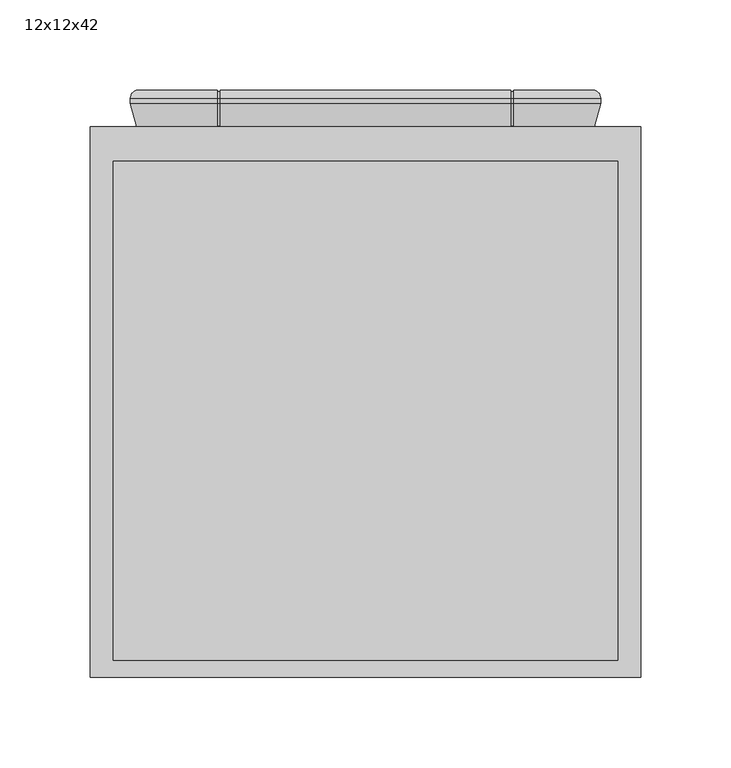
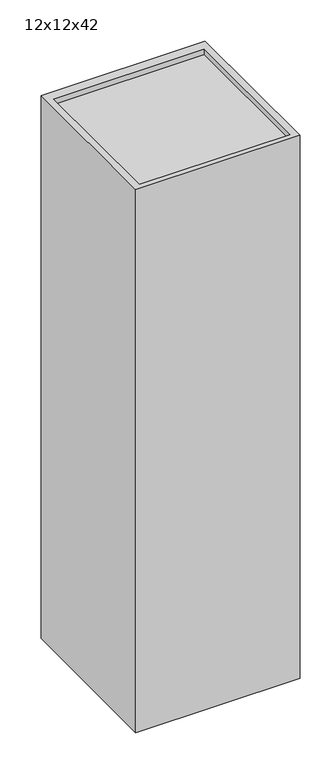
"""IFC4 building model written with IfcOpenShell, lengths in millimetres: furniture geometry, Cabinet-Wall-Merillat-Single_Door-Marlin : 12x12x42."""

from ifc_helpers import new_model, si_unit, frame, origin, place, context, project, spatial, polyline, circle_curve, ellipse_curve, outline, extrude, faceted_brep, source, transform, mapped, element, save
from ifc_brep_helpers import plane_surface, cylinder_surface, advanced_brep


def furniture_12x12x42_3f69c235(model_context):
    return source(origin(), model_context, "Body", "SolidModel", [
        advanced_brep(
        [(-100.4038372, 382.5621, 2108.2), (-97.3073447, 387.0325, 2105.1035075), (-97.3073447, 387.0325, 1095.2964925), (-100.4038372, 382.5621, 1092.2), (-100.4038372, 379.7935, 1092.2), (-100.4038372, 379.7935, 2108.2), (-96.8986372, 366.7125, 1095.7052), (-96.8986372, 366.7125, 2104.6948), (-52.2026744, 366.7125, 2059.9988372), (-52.2026744, 366.7125, 1140.4011628), (-51.8325427, 367.50625, 1140.7712945), (-49.7513837, 371.96931, 1142.8524535), (-49.7513837, 371.96931, 2057.5475465), (-51.8325427, 367.50625, 2059.6287055), (-51.1511532, 374.2094093, 1141.452684), (-51.1511532, 374.2094093, 2058.947316), (-65.4788372, 374.4595, 1127.125), (-65.4788372, 374.4595, 2073.275), (-65.4788372, 379.2855, 1127.125), (-65.4788372, 379.2855, 2073.275), (-51.1511532, 379.5355907, 1141.452684), (-51.1511532, 379.5355907, 2058.947316), (-49.7513837, 381.77569, 1142.8524535), (-49.7513837, 381.77569, 2057.5475465), (-51.8325427, 386.23875, 1140.7712945), (-52.199807, 387.0263508, 1140.4040302), (-52.2026744, 387.0325, 2059.9988372), (-51.8325427, 386.23875, 2059.6287055), (-52.199807, 387.0325, 1095.2964925), (-52.199807, 382.5621, 1092.2), (156.8496703, 387.0325, 1095.2964925), (159.9461628, 382.5621, 1092.2), (111.7819441, 382.5621, 1092.2), (111.7819441, 387.0325, 1095.2964925), (-50.612307, 382.5621, 1092.2), (-50.612307, 387.0325, 1095.2964925), (110.1944441, 387.0325, 1095.2964925), (110.1944441, 382.5621, 1092.2), (-52.199807, 379.7935, 1092.2), (159.9461628, 379.7935, 1092.2), (111.7819441, 379.7935, 1092.2), (-50.612307, 379.7935, 1092.2), (110.1944441, 379.7935, 1092.2), (-52.199807, 366.7125, 1095.7052), (156.4409628, 366.7125, 1095.7052), (111.7819441, 366.7125, 1095.7052), (-50.612307, 366.7125, 1095.7052), (110.1944441, 366.7125, 1095.7052), (109.2937093, 371.96931, 1142.8524535), (-50.612307, 367.50625, 1140.7712945), (-50.612307, 366.7125, 1140.4011628), (110.1944441, 366.7125, 1140.4011628), (110.1944441, 367.50625, 1140.7712945), (111.3748683, 367.50625, 1140.7712945), (110.6934787, 374.2094093, 1141.452684), (125.0211628, 374.4595, 1127.125), (125.0211628, 379.2855, 1127.125), (110.6934787, 379.5355907, 1141.452684), (109.2937093, 381.77569, 1142.8524535), (111.3748683, 386.23875, 1140.7712945), (110.1944441, 386.23875, 1140.7712945), (110.1944441, 387.0325, 1140.4011628), (-50.612307, 387.0325, 1140.4011628), (-50.612307, 386.23875, 1140.7712945), (156.8496703, 387.0325, 2105.1035075), (159.9461628, 382.5621, 2108.2), (159.9461628, 379.7935, 2108.2), (156.4409628, 366.7125, 2104.6948), (111.745, 366.7125, 1140.4011628), (111.745, 366.7125, 2059.9988372), (111.3748683, 367.50625, 2059.6287055), (109.2937093, 371.96931, 2057.5475465), (110.6934787, 374.2094093, 2058.947316), (125.0211628, 374.4595, 2073.275), (125.0211628, 379.2855, 2073.275), (110.6934787, 379.5355907, 2058.947316), (109.2937093, 381.77569, 2057.5475465), (111.3748683, 386.23875, 2059.6287055), (111.745, 387.0325, 2059.9988372), (111.745, 387.0325, 1140.4011628), (111.7819441, 387.0325, 2105.1035075), (111.7819441, 382.5621, 2108.2), (-52.199807, 382.5621, 2108.2), (-52.199807, 387.0325, 2105.1035075), (110.1944441, 382.5621, 2108.2), (110.1944441, 387.0325, 2105.1035075), (-50.612307, 387.0325, 2105.1035075), (-50.612307, 382.5621, 2108.2), (111.7819441, 379.7935, 2108.2), (-52.199807, 379.7935, 2108.2), (110.1944441, 379.7935, 2108.2), (-50.612307, 379.7935, 2108.2), (111.7819441, 366.7125, 2104.6948), (-52.199807, 366.7125, 2104.6948), (110.1944441, 366.7125, 2104.6948), (-50.612307, 366.7125, 2104.6948), (110.1944441, 366.7125, 2059.9988372), (-50.612307, 366.7125, 2059.9988372), (110.1944441, 367.50625, 2059.6287055), (-50.612307, 367.50625, 2059.6287055), (-50.612307, 386.23875, 2059.6287055), (-50.612307, 387.0325, 2059.9988372), (110.1944441, 387.0325, 2059.9988372), (110.1944441, 386.23875, 2059.6287055), (110.1944441, 367.50625, 2104.0857412), (110.1944441, 379.8980037, 2107.40625), (110.1944441, 382.5621, 2107.40625), (110.1944441, 386.23875, 2104.9526052), (111.7819441, 386.23875, 2059.6287055), (111.7819441, 386.23875, 2104.9526052), (111.7819441, 382.5621, 2107.40625), (111.7819441, 379.8980037, 2107.40625), (111.7819441, 367.50625, 2104.0857412), (111.7819441, 367.50625, 2059.6287055), (-52.199807, 367.50625, 2059.6287055), (-52.199807, 367.50625, 2104.0857412), (-52.199807, 379.8980037, 2107.40625), (-52.199807, 382.5621, 2107.40625), (-52.199807, 386.23875, 2104.9526052), (-52.199807, 386.23875, 2059.6287055), (-50.612307, 386.23875, 2104.9526052), (-50.612307, 382.5621, 2107.40625), (-50.612307, 379.8980037, 2107.40625), (-50.612307, 367.50625, 2104.0857412), (-52.199807, 386.23875, 1140.7712945), (-52.199807, 386.23875, 1095.4473948), (-52.199807, 382.5621, 1092.99375), (-52.199807, 379.8980037, 1092.99375), (-52.199807, 367.50625, 1096.3142588), (-52.199807, 367.50625, 1140.7712945), (-50.612307, 367.50625, 1096.3142588), (-50.612307, 379.8980037, 1092.99375), (-50.612307, 382.5621, 1092.99375), (-50.612307, 386.23875, 1095.4473948), (110.1944441, 386.23875, 1095.4473948), (110.1944441, 382.5621, 1092.99375), (110.1944441, 379.8980037, 1092.99375), (110.1944441, 367.50625, 1096.3142588), (111.7819441, 386.23875, 1140.7712945), (111.7819441, 367.50625, 1140.7712945), (111.7819441, 367.50625, 1096.3142588), (111.7819441, 379.8980037, 1092.99375), (111.7819441, 382.5621, 1092.99375), (111.7819441, 386.23875, 1095.4473948)],
        [
            (0, 1, ellipse_curve(frame((-95.6286372, 382.5621, 2103.4248), z_axis=(-0.7071067811865475, 0.0, -0.7071067811865475), x_axis=(-0.7071067811865474, 0.0, 0.7071067811865476)), 6.7531526, 4.7752)),
            (1, 2),
            (2, 3, ellipse_curve(frame((-95.6286372, 382.5621, 1096.9752), z_axis=(-0.7071067811865475, 0.0, 0.7071067811865475), x_axis=(0.7071067811865474, 0.0, 0.7071067811865476)), 6.7531526, 4.7752)),
            (3, 0),
            (3, 4),
            (4, 5),
            (5, 0),
            (4, 6),
            (6, 7),
            (7, 5),
            (8, 9),
            (9, 10),
            (10, 11),
            (11, 12),
            (12, 13),
            (13, 8),
            (11, 14, ellipse_curve(frame((-51.1786372, 372.6348492, 1141.4252), z_axis=(-0.7071067811865475, 0.0, 0.7071067811865475), x_axis=(0.7071067811865474, 0.0, 0.7071067811865476)), 2.2271035, 1.5748)),
            (14, 15),
            (15, 12, ellipse_curve(frame((-51.1786372, 372.6348492, 2058.9748), z_axis=(-0.7071067811865475, 0.0, -0.7071067811865475), x_axis=(-0.7071067811865474, 0.0, 0.7071067811865476)), 2.2271035, 1.5748)),
            (14, 16),
            (16, 17),
            (17, 15),
            (16, 18),
            (18, 19),
            (19, 17),
            (18, 20),
            (20, 21),
            (21, 19),
            (20, 22, ellipse_curve(frame((-51.1786372, 381.1101508, 1141.4252), z_axis=(-0.7071067811865475, 0.0, 0.7071067811865475), x_axis=(0.7071067811865474, 0.0, 0.7071067811865476)), 2.2271035, 1.5748)),
            (22, 23),
            (23, 21, ellipse_curve(frame((-51.1786372, 381.1101508, 2058.9748), z_axis=(-0.7071067811865475, 0.0, -0.7071067811865475), x_axis=(-0.7071067811865474, 0.0, 0.7071067811865476)), 2.2271035, 1.5748)),
            (22, 24),
            (24, 25),
            (25, 26),
            (26, 27),
            (27, 23),
            (2, 28),
            (28, 29, circle_curve(frame((-52.199807, 382.5621, 1096.9752), z_axis=(-1.0, 0.0, 0.0), x_axis=(0.0, -1.0, 0.0)), 4.7752)),
            (29, 3),
            (30, 31, ellipse_curve(frame((155.1709628, 382.5621, 1096.9752), z_axis=(-0.7071067811865475, 0.0, -0.7071067811865475), x_axis=(-0.7071067811865476, 0.0, 0.7071067811865474)), 6.7531526, 4.7752)),
            (31, 32),
            (32, 33, circle_curve(frame((111.7819441, 382.5621, 1096.9752), z_axis=(1.0, 0.0, 0.0), x_axis=(0.0, -1.0, 0.0)), 4.7752)),
            (33, 30),
            (34, 35, circle_curve(frame((-50.612307, 382.5621, 1096.9752), z_axis=(1.0, 0.0, 0.0), x_axis=(0.0, -1.0, 0.0)), 4.7752)),
            (35, 36),
            (36, 37, circle_curve(frame((110.1944441, 382.5621, 1096.9752), z_axis=(-1.0, 0.0, 0.0), x_axis=(0.0, -1.0, 0.0)), 4.7752)),
            (37, 34),
            (29, 38),
            (38, 4),
            (31, 39),
            (39, 40),
            (40, 32),
            (41, 34),
            (37, 42),
            (42, 41),
            (38, 43),
            (43, 6),
            (39, 44),
            (44, 45),
            (45, 40),
            (46, 41),
            (42, 47),
            (47, 46),
            (48, 11),
            (10, 49),
            (49, 50),
            (50, 51),
            (51, 52),
            (52, 53),
            (53, 48),
            (48, 54, ellipse_curve(frame((110.7209628, 372.6348492, 1141.4252), z_axis=(-0.7071067811865475, 0.0, -0.7071067811865475), x_axis=(-0.7071067811865476, 0.0, 0.7071067811865474)), 2.2271035, 1.5748)),
            (54, 14),
            (54, 55),
            (55, 16),
            (55, 56),
            (56, 18),
            (56, 57),
            (57, 20),
            (57, 58, ellipse_curve(frame((110.7209628, 381.1101508, 1141.4252), z_axis=(-0.7071067811865475, 0.0, -0.7071067811865475), x_axis=(-0.7071067811865476, 0.0, 0.7071067811865474)), 2.2271035, 1.5748)),
            (58, 22),
            (58, 59),
            (59, 60),
            (60, 61),
            (61, 62),
            (62, 63),
            (63, 24),
            (30, 64),
            (64, 65, ellipse_curve(frame((155.1709628, 382.5621, 2103.4248), z_axis=(0.7071067811865475, 0.0, -0.7071067811865475), x_axis=(-0.7071067811865474, 0.0, -0.7071067811865476)), 6.7531526, 4.7752)),
            (65, 31),
            (65, 66),
            (66, 39),
            (66, 67),
            (67, 44),
            (68, 69),
            (69, 70),
            (70, 71),
            (71, 48),
            (53, 68),
            (71, 72, ellipse_curve(frame((110.7209628, 372.6348492, 2058.9748), z_axis=(0.7071067811865475, 0.0, -0.7071067811865475), x_axis=(-0.7071067811865474, 0.0, -0.7071067811865476)), 2.2271035, 1.5748)),
            (72, 54),
            (72, 73),
            (73, 55),
            (73, 74),
            (74, 56),
            (74, 75),
            (75, 57),
            (75, 76, ellipse_curve(frame((110.7209628, 381.1101508, 2058.9748), z_axis=(0.7071067811865475, 0.0, -0.7071067811865475), x_axis=(-0.7071067811865474, 0.0, -0.7071067811865476)), 2.2271035, 1.5748)),
            (76, 58),
            (76, 77),
            (77, 78),
            (78, 79),
            (79, 59),
            (64, 80),
            (80, 81, circle_curve(frame((111.7819441, 382.5621, 2103.4248), z_axis=(1.0, 0.0, 0.0), x_axis=(0.0, -1.0, 0.0)), 4.7752)),
            (81, 65),
            (0, 82),
            (82, 83, circle_curve(frame((-52.199807, 382.5621, 2103.4248), z_axis=(-1.0, 0.0, 0.0), x_axis=(0.0, -1.0, 0.0)), 4.7752)),
            (83, 1),
            (84, 85, circle_curve(frame((110.1944441, 382.5621, 2103.4248), z_axis=(-1.0, 0.0, 0.0), x_axis=(0.0, -1.0, 0.0)), 4.7752)),
            (85, 86),
            (86, 87, circle_curve(frame((-50.612307, 382.5621, 2103.4248), z_axis=(1.0, 0.0, 0.0), x_axis=(0.0, -1.0, 0.0)), 4.7752)),
            (87, 84),
            (81, 88),
            (88, 66),
            (5, 89),
            (89, 82),
            (90, 84),
            (87, 91),
            (91, 90),
            (88, 92),
            (92, 67),
            (7, 93),
            (93, 89),
            (94, 90),
            (91, 95),
            (95, 94),
            (43, 9),
            (8, 93),
            (92, 69),
            (68, 45),
            (96, 94),
            (95, 97),
            (97, 96),
            (50, 46),
            (47, 51),
            (12, 71),
            (70, 98),
            (98, 96),
            (97, 99),
            (99, 13),
            (15, 72),
            (17, 73),
            (19, 74),
            (21, 75),
            (23, 76),
            (27, 100),
            (100, 101),
            (101, 102),
            (102, 103),
            (103, 77),
            (83, 26),
            (25, 28),
            (33, 79),
            (78, 80),
            (85, 102),
            (101, 86),
            (35, 62),
            (61, 36),
            (98, 104),
            (104, 105),
            (105, 106),
            (106, 107, circle_curve(frame((110.1944441, 382.5621, 2103.4248), z_axis=(-1.0, 0.0, 0.0), x_axis=(0.0, 0.0, 1.0)), 3.98145)),
            (107, 103),
            (78, 108),
            (108, 109),
            (109, 110, circle_curve(frame((111.7819441, 382.5621, 2103.4248), z_axis=(1.0, 0.0, 0.0), x_axis=(0.0, 0.0, 1.0)), 3.98145)),
            (110, 111),
            (111, 112),
            (112, 113),
            (113, 69),
            (77, 108),
            (107, 109),
            (106, 110),
            (105, 111),
            (104, 112),
            (70, 113),
            (8, 114),
            (114, 115),
            (115, 116),
            (116, 117),
            (117, 118, circle_curve(frame((-52.199807, 382.5621, 2103.4248), z_axis=(-1.0, 0.0, 0.0), x_axis=(0.0, 0.0, 1.0)), 3.98145)),
            (118, 119),
            (119, 26),
            (100, 120),
            (120, 121, circle_curve(frame((-50.612307, 382.5621, 2103.4248), z_axis=(1.0, 0.0, 0.0), x_axis=(0.0, 0.0, 1.0)), 3.98145)),
            (121, 122),
            (122, 123),
            (123, 99),
            (119, 27),
            (118, 120),
            (117, 121),
            (116, 122),
            (115, 123),
            (114, 13),
            (25, 124),
            (124, 125),
            (125, 126, circle_curve(frame((-52.199807, 382.5621, 1096.9752), z_axis=(-1.0, 0.0, 0.0), x_axis=(0.0, 0.0, 1.0)), 3.98145)),
            (126, 127),
            (127, 128),
            (128, 129),
            (129, 9),
            (49, 130),
            (130, 131),
            (131, 132),
            (132, 133, circle_curve(frame((-50.612307, 382.5621, 1096.9752), z_axis=(1.0, 0.0, 0.0), x_axis=(0.0, 0.0, 1.0)), 3.98145)),
            (133, 63),
            (129, 10),
            (128, 130),
            (127, 131),
            (126, 132),
            (125, 133),
            (124, 24),
            (60, 134),
            (134, 135, circle_curve(frame((110.1944441, 382.5621, 1096.9752), z_axis=(-1.0, 0.0, 0.0), x_axis=(0.0, 0.0, 1.0)), 3.98145)),
            (135, 136),
            (136, 137),
            (137, 52),
            (138, 79),
            (68, 139),
            (139, 140),
            (140, 141),
            (141, 142),
            (142, 143, circle_curve(frame((111.7819441, 382.5621, 1096.9752), z_axis=(1.0, 0.0, 0.0), x_axis=(0.0, 0.0, 1.0)), 3.98145)),
            (143, 138),
            (138, 59),
            (53, 139),
            (137, 140),
            (136, 141),
            (135, 142),
            (134, 143),
        ],
        [
            cylinder_surface(frame((-95.6286372, 382.5621, 2108.2), z_axis=(0.0, 0.0, 1.0), x_axis=(0.0, -1.0, 0.0)), 4.7752),
            plane_surface(frame((-100.4038372, 382.5621, 2108.2), z_axis=(-1.0, 0.0, 0.0), x_axis=(0.0, 0.0, -1.0))),
            plane_surface(frame((-100.4038372, 379.7935, 2108.2), z_axis=(-0.9659229350723619, -0.25882983502910506, 0.0), x_axis=(0.0, 0.0, -1.0))),
            plane_surface(frame((-52.2026744, 366.7125, 2059.9988372), z_axis=(0.9063077870366099, -0.4226182617407856, 0.0), x_axis=(0.0, 0.0, -1.0))),
            cylinder_surface(frame((-51.1786372, 372.6348492, 2108.2), z_axis=(0.0, 0.0, 1.0000000000000002), x_axis=(0.01745240643729364, 0.9998476951563912, 0.0)), 1.5748),
            plane_surface(frame((-51.1511532, 374.2094093, 2058.947316), z_axis=(0.017452406437322144, 0.9998476951563906, 0.0), x_axis=(0.0, 0.0, -1.0))),
            plane_surface(frame((-65.4788372, 374.4595, 2073.275), z_axis=(1.0, 0.0, 0.0), x_axis=(0.0, 0.0, -1.0))),
            plane_surface(frame((-65.4788372, 379.2855, 2073.275), z_axis=(0.01745240643727848, -0.9998476951563914, 0.0), x_axis=(0.0, 0.0, -1.0))),
            cylinder_surface(frame((-51.1786372, 381.1101508, 2108.2), z_axis=(0.0, 0.0, 1.0000000000000002), x_axis=(0.9063077870367326, 0.42261826174052236, 0.0)), 1.5748),
            plane_surface(frame((-49.7513837, 381.77569, 2057.5475465), z_axis=(0.9063077870366333, 0.4226182617407352, 0.0), x_axis=(0.0, 0.0, -1.0))),
            cylinder_surface(frame((-100.4038372, 382.5621, 1096.9752), z_axis=(-1.0, 0.0, 0.0), x_axis=(0.0, -1.0, 0.0)), 4.7752),
            plane_surface(frame((-100.4038372, 382.5621, 1092.2), z_axis=(0.0, 0.0, -1.0), x_axis=(1.0, 0.0, 0.0))),
            plane_surface(frame((-100.4038372, 379.7935, 1092.2), z_axis=(0.0, -0.2588298350291095, -0.9659229350723607), x_axis=(1.0, 0.0, 0.0))),
            plane_surface(frame((-52.2026744, 366.7125, 1140.4011628), z_axis=(0.0, -0.42261826174078143, 0.9063077870366119), x_axis=(1.0, 0.0, 0.0))),
            cylinder_surface(frame((-100.4038372, 372.6348492, 1141.4252), z_axis=(-1.0000000000000002, 0.0, 0.0), x_axis=(0.0, 0.9998476951563913, 0.017452406437289025)), 1.5748),
            plane_surface(frame((-51.1511532, 374.2094093, 1141.452684), z_axis=(0.0, 0.9998476951563907, 0.01745240643731753), x_axis=(1.0, 0.0, 0.0))),
            plane_surface(frame((-65.4788372, 374.4595, 1127.125), z_axis=(0.0, 0.0, 1.0), x_axis=(1.0, 0.0, 0.0))),
            plane_surface(frame((-65.4788372, 379.2855, 1127.125), z_axis=(0.0, -0.9998476951563913, 0.017452406437283095), x_axis=(1.0, 0.0, 0.0))),
            cylinder_surface(frame((-100.4038372, 381.1101508, 1141.4252), z_axis=(-1.0000000000000002, 0.0, 0.0), x_axis=(0.0, 0.4226182617405265, 0.9063077870367306)), 1.5748),
            plane_surface(frame((-49.7513837, 381.77569, 1142.8524535), z_axis=(0.0, 0.4226182617407394, 0.9063077870366314), x_axis=(1.0, 0.0, 0.0))),
            cylinder_surface(frame((155.1709628, 382.5621, 1092.2), z_axis=(0.0, 0.0, -1.0), x_axis=(0.0, -1.0, 0.0)), 4.7752),
            plane_surface(frame((159.9461628, 382.5621, 1092.2), z_axis=(1.0, 0.0, 0.0), x_axis=(0.0, 0.0, 1.0))),
            plane_surface(frame((159.9461628, 379.7935, 1092.2), z_axis=(0.9659229350723619, -0.25882983502910506, 0.0), x_axis=(0.0, 0.0, 1.0))),
            plane_surface(frame((111.745, 366.7125, 1140.4011628), z_axis=(-0.9063077870366099, -0.4226182617407856, 0.0), x_axis=(0.0, 0.0, 1.0))),
            cylinder_surface(frame((110.7209628, 372.6348492, 1092.2), z_axis=(0.0, 0.0, -1.0000000000000002), x_axis=(-0.01745240643729364, 0.9998476951563912, 0.0)), 1.5748),
            plane_surface(frame((110.6934787, 374.2094093, 1141.452684), z_axis=(-0.017452406437322144, 0.9998476951563906, 0.0), x_axis=(0.0, 0.0, 1.0))),
            plane_surface(frame((125.0211628, 374.4595, 1127.125), z_axis=(-1.0, 0.0, 0.0), x_axis=(0.0, 0.0, 1.0))),
            plane_surface(frame((125.0211628, 379.2855, 1127.125), z_axis=(-0.01745240643727848, -0.9998476951563914, 0.0), x_axis=(0.0, 0.0, 1.0))),
            cylinder_surface(frame((110.7209628, 381.1101508, 1092.2), z_axis=(0.0, 0.0, -1.0000000000000002), x_axis=(-0.9063077870367326, 0.42261826174052236, 0.0)), 1.5748),
            plane_surface(frame((109.2937093, 381.77569, 1142.8524535), z_axis=(-0.9063077870366333, 0.4226182617407352, 0.0), x_axis=(0.0, 0.0, 1.0))),
            cylinder_surface(frame((159.9461628, 382.5621, 2103.4248), z_axis=(1.0, 0.0, 0.0), x_axis=(0.0, -1.0, 0.0)), 4.7752),
            plane_surface(frame((159.9461628, 382.5621, 2108.2), z_axis=(0.0, 0.0, 1.0), x_axis=(-1.0, 0.0, 0.0))),
            plane_surface(frame((159.9461628, 379.7935, 2108.2), z_axis=(0.0, -0.2588298350291006, 0.9659229350723632), x_axis=(-1.0, 0.0, 0.0))),
            plane_surface(frame((156.4409628, 366.7125, 2104.6948), z_axis=(0.0, -1.0, 0.0), x_axis=(-1.0, 0.0, 0.0))),
            plane_surface(frame((111.745, 366.7125, 2059.9988372), z_axis=(0.0, -0.42261826174078976, -0.9063077870366079), x_axis=(-1.0, 0.0, 0.0))),
            cylinder_surface(frame((159.9461628, 372.6348492, 2058.9748), z_axis=(1.0000000000000002, 0.0, 0.0), x_axis=(0.0, 0.999847695156391, -0.017452406437298253)), 1.5748),
            plane_surface(frame((110.6934787, 374.2094093, 2058.947316), z_axis=(0.0, 0.9998476951563905, -0.01745240643732676), x_axis=(-1.0, 0.0, 0.0))),
            plane_surface(frame((125.0211628, 374.4595, 2073.275), z_axis=(0.0, 0.0, -1.0), x_axis=(-1.0, 0.0, 0.0))),
            plane_surface(frame((125.0211628, 379.2855, 2073.275), z_axis=(0.0, -0.9998476951563915, -0.017452406437273867), x_axis=(-1.0, 0.0, 0.0))),
            cylinder_surface(frame((159.9461628, 381.1101508, 2058.9748), z_axis=(1.0000000000000002, 0.0, 0.0), x_axis=(0.0, 0.4226182617405182, -0.9063077870367346)), 1.5748),
            plane_surface(frame((109.2937093, 381.77569, 2057.5475465), z_axis=(0.0, 0.422618261740731, -0.9063077870366353), x_axis=(-1.0, 0.0, 0.0))),
            plane_surface(frame((111.745, 387.0325, 2059.9988372), z_axis=(0.0, 1.0, 0.0), x_axis=(-1.0, 0.0, 0.0))),
            plane_surface(frame((110.1944441, 387.0325, 2059.9988372), z_axis=(1.0, 0.0, 0.0), x_axis=(0.0, -0.9063077870366119, -0.4226182617407812))),
            plane_surface(frame((111.7819441, 387.0325, 2059.9988372), z_axis=(-1.0, 0.0, 0.0), x_axis=(0.0, 0.9063077870366119, 0.4226182617407812))),
            plane_surface(frame((110.1944441, 387.0325, 2059.9988372), z_axis=(0.0, -0.4226182617407812, 0.9063077870366119), x_axis=(1.0, 0.0, 0.0))),
            plane_surface(frame((110.1944441, 386.23875, 2059.6287055), z_axis=(0.0, 1.0, 0.0), x_axis=(1.0, 0.0, 0.0))),
            cylinder_surface(frame((111.7819441, 382.5621, 2103.4248), z_axis=(1.0, 0.0, 0.0), x_axis=(0.0, 0.0, 1.0)), 3.98145),
            plane_surface(frame((110.1944441, 382.5621, 2107.40625), z_axis=(0.0, 0.0, 1.0), x_axis=(1.0, 0.0, 0.0))),
            plane_surface(frame((110.1944441, 379.8980037, 2107.40625), z_axis=(0.0, -0.25882983502916007, 0.9659229350723473), x_axis=(1.0, 0.0, 0.0))),
            plane_surface(frame((110.1944441, 367.50625, 2104.0857412), z_axis=(0.0, -1.0, 0.0), x_axis=(1.0, 0.0, 0.0))),
            plane_surface(frame((110.1944441, 367.50625, 2059.6287055), z_axis=(0.0, 0.4226182617408151, 0.906307787036596), x_axis=(1.0, 0.0, 0.0))),
            plane_surface(frame((-52.199807, 387.0325, 2059.9988372), z_axis=(1.0, 0.0, 0.0), x_axis=(0.0, -0.9063077870366119, -0.4226182617407812))),
            plane_surface(frame((-50.612307, 387.0325, 2059.9988372), z_axis=(-1.0, 0.0, 0.0), x_axis=(0.0, 0.9063077870366119, 0.4226182617407812))),
            plane_surface(frame((-52.199807, 387.0325, 2059.9988372), z_axis=(0.0, -0.4226182617407812, 0.9063077870366119), x_axis=(1.0, 0.0, 0.0))),
            plane_surface(frame((-52.199807, 386.23875, 2059.6287055), z_axis=(0.0, 1.0, 0.0), x_axis=(1.0, 0.0, 0.0))),
            cylinder_surface(frame((-50.612307, 382.5621, 2103.4248), z_axis=(1.0, 0.0, 0.0), x_axis=(0.0, 0.0, 1.0)), 3.98145),
            plane_surface(frame((-52.199807, 382.5621, 2107.40625), z_axis=(0.0, 0.0, 1.0), x_axis=(1.0, 0.0, 0.0))),
            plane_surface(frame((-52.199807, 379.8980037, 2107.40625), z_axis=(0.0, -0.25882983502916257, 0.9659229350723466), x_axis=(1.0, 0.0, 0.0))),
            plane_surface(frame((-52.199807, 367.50625, 2104.0857412), z_axis=(0.0, -1.0, 0.0), x_axis=(1.0, 0.0, 0.0))),
            plane_surface(frame((-52.199807, 367.50625, 2059.6287055), z_axis=(0.0, 0.42261826174081607, 0.9063077870365956), x_axis=(1.0, 0.0, 0.0))),
            plane_surface(frame((-52.199807, 382.5621, 1101.7504), z_axis=(1.0, 0.0, 0.0), x_axis=(0.0, 1.0, 0.0))),
            plane_surface(frame((-50.612307, 382.5621, 1101.7504), z_axis=(-1.0, 0.0, 0.0), x_axis=(0.0, -1.0, 0.0))),
            plane_surface(frame((-52.199807, 366.7125, 1140.4011628), z_axis=(0.0, 0.4226182617407898, -0.906307787036608), x_axis=(1.0, 0.0, 0.0))),
            plane_surface(frame((-52.199807, 367.50625, 1140.7712945), z_axis=(0.0, -1.0, 0.0), x_axis=(1.0, 0.0, 0.0))),
            plane_surface(frame((-52.199807, 367.50625, 1096.3142588), z_axis=(0.0, -0.2588298350294553, -0.9659229350722681), x_axis=(1.0, 0.0, 0.0))),
            plane_surface(frame((-52.199807, 379.8980037, 1092.99375), z_axis=(0.0, 0.0, -1.0), x_axis=(1.0, 0.0, 0.0))),
            cylinder_surface(frame((-50.612307, 382.5621, 1096.9752), z_axis=(1.0, 0.0, 0.0), x_axis=(0.0, 0.0, 1.0)), 3.98145),
            plane_surface(frame((-52.199807, 386.23875, 1095.4473948), z_axis=(0.0, 1.0, 0.0), x_axis=(1.0, 0.0, 0.0))),
            plane_surface(frame((-52.199807, 386.23875, 1140.7712945), z_axis=(0.0, -0.42261826174079614, -0.9063077870366049), x_axis=(1.0, 0.0, 0.0))),
            plane_surface(frame((110.1944441, 386.23875, 1140.7712945), z_axis=(1.0000000000000002, 0.0, 0.0), x_axis=(0.0, 0.9063077870366271, -0.4226182617407486))),
            plane_surface(frame((111.7819441, 386.23875, 1140.7712945), z_axis=(-1.0000000000000002, 0.0, 0.0), x_axis=(0.0, -0.9063077870366271, 0.4226182617407486))),
            plane_surface(frame((110.1944441, 386.23875, 1140.7712945), z_axis=(0.0, -0.4226182617407486, -0.9063077870366271), x_axis=(1.0, 0.0, 0.0))),
            plane_surface(frame((110.1944441, 366.7125, 1140.4011628), z_axis=(0.0, 0.4226182617407898, -0.906307787036608), x_axis=(1.0, 0.0, 0.0))),
            plane_surface(frame((110.1944441, 367.50625, 1140.7712945), z_axis=(0.0, -1.0, 0.0), x_axis=(1.0, 0.0, 0.0))),
            plane_surface(frame((110.1944441, 367.50625, 1096.3142588), z_axis=(0.0, -0.25882983502945534, -0.9659229350722681), x_axis=(1.0, 0.0, 0.0))),
            plane_surface(frame((110.1944441, 379.8980037, 1092.99375), z_axis=(0.0, 0.0, -1.0), x_axis=(1.0, 0.0, 0.0))),
            cylinder_surface(frame((111.7819441, 382.5621, 1096.9752), z_axis=(1.0, 0.0, 0.0), x_axis=(0.0, 0.0, 1.0)), 3.98145),
            plane_surface(frame((110.1944441, 386.23875, 1095.4473948), z_axis=(0.0, 1.0, 0.0), x_axis=(1.0, 0.0, 0.0))),
        ],
        [
            (0, [[1, 2, 3, 4]]),
            (1, [[-4, 5, 6, 7]]),
            (2, [[-6, 8, 9, 10]]),
            (3, [[11, 12, 13, 14, 15, 16]]),
            (4, [[-14, 17, 18, 19]]),
            (5, [[-18, 20, 21, 22]]),
            (6, [[-21, 23, 24, 25]]),
            (7, [[-24, 26, 27, 28]]),
            (8, [[-27, 29, 30, 31]]),
            (9, [[-30, 32, 33, 34, 35, 36]]),
            (10, [[-3, 37, 38, 39]]),
            (10, [[40, 41, 42, 43]]),
            (10, [[44, 45, 46, 47]]),
            (11, [[-5, -39, 48, 49]]),
            (11, [[50, 51, 52, -41]]),
            (11, [[53, -47, 54, 55]]),
            (12, [[-8, -49, 56, 57]]),
            (12, [[58, 59, 60, -51]]),
            (12, [[61, -55, 62, 63]]),
            (13, [[64, -13, 65, 66, 67, 68, 69, 70]]),
            (14, [[-17, -64, 71, 72]]),
            (15, [[-20, -72, 73, 74]]),
            (16, [[-23, -74, 75, 76]]),
            (17, [[-26, -76, 77, 78]]),
            (18, [[-29, -78, 79, 80]]),
            (19, [[-80, 81, 82, 83, 84, 85, 86, -32]]),
            (20, [[-40, 87, 88, 89]]),
            (21, [[-50, -89, 90, 91]]),
            (22, [[-58, -91, 92, 93]]),
            (23, [[94, 95, 96, 97, -70, 98]]),
            (24, [[-71, -97, 99, 100]]),
            (25, [[-73, -100, 101, 102]]),
            (26, [[-75, -102, 103, 104]]),
            (27, [[-77, -104, 105, 106]]),
            (28, [[-79, -106, 107, 108]]),
            (29, [[-108, 109, 110, 111, 112, -81]]),
            (30, [[-88, 113, 114, 115]]),
            (30, [[-1, 116, 117, 118]]),
            (30, [[119, 120, 121, 122]]),
            (31, [[-90, -115, 123, 124]]),
            (31, [[-7, 125, 126, -116]]),
            (31, [[127, -122, 128, 129]]),
            (32, [[-92, -124, 130, 131]]),
            (32, [[-10, 132, 133, -125]]),
            (32, [[134, -129, 135, 136]]),
            (33, [[-9, -57, 137, -11, 138, -132]]),
            (33, [[-93, -131, 139, -94, 140, -59]]),
            (33, [[141, -136, 142, 143]]),
            (33, [[144, -63, 145, -67]]),
            (34, [[146, -96, 147, 148, -143, 149, 150, -15]]),
            (35, [[-19, 151, -99, -146]]),
            (36, [[-22, 152, -101, -151]]),
            (37, [[-25, 153, -103, -152]]),
            (38, [[-28, 154, -105, -153]]),
            (39, [[-31, 155, -107, -154]]),
            (40, [[-155, -36, 156, 157, 158, 159, 160, -109]]),
            (41, [[-2, -118, 161, -34, 162, -37]]),
            (41, [[-87, -43, 163, -111, 164, -113]]),
            (41, [[165, -158, 166, -120]]),
            (41, [[167, -84, 168, -45]]),
            (42, [[169, 170, 171, 172, 173, -159, -165, -119, -127, -134, -141, -148]]),
            (43, [[174, 175, 176, 177, 178, 179, 180, -139, -130, -123, -114, -164]]),
            (44, [[-174, -110, 181]]),
            (45, [[-173, 182, -175, -181, -160]]),
            (46, [[-172, 183, -176, -182]]),
            (47, [[-171, 184, -177, -183]]),
            (48, [[-170, 185, -178, -184]]),
            (49, [[-169, -147, 186, -179, -185]]),
            (50, [[-180, -186, -95]]),
            (51, [[187, 188, 189, 190, 191, 192, 193, -161, -117, -126, -133, -138]]),
            (52, [[194, 195, 196, 197, 198, -149, -142, -135, -128, -121, -166, -157]]),
            (53, [[-193, 199, -35]]),
            (54, [[-192, 200, -194, -156, -199]]),
            (55, [[-191, 201, -195, -200]]),
            (56, [[-190, 202, -196, -201]]),
            (57, [[-189, 203, -197, -202]]),
            (58, [[-188, 204, -150, -198, -203]]),
            (59, [[-187, -16, -204]]),
            (60, [[205, 206, 207, 208, 209, 210, 211, -137, -56, -48, -38, -162]]),
            (61, [[212, 213, 214, 215, 216, -85, -167, -44, -53, -61, -144, -66]]),
            (62, [[-211, 217, -12]]),
            (63, [[-210, 218, -212, -65, -217]]),
            (64, [[-209, 219, -213, -218]]),
            (65, [[-208, 220, -214, -219]]),
            (66, [[-207, 221, -215, -220]]),
            (67, [[-206, 222, -86, -216, -221]]),
            (68, [[-205, -33, -222]]),
            (69, [[223, 224, 225, 226, 227, -68, -145, -62, -54, -46, -168, -83]]),
            (70, [[228, -163, -42, -52, -60, -140, 229, 230, 231, 232, 233, 234]]),
            (71, [[-228, 235, -112]]),
            (72, [[-229, -98, 236]]),
            (73, [[-227, 237, -230, -236, -69]]),
            (74, [[-226, 238, -231, -237]]),
            (75, [[-225, 239, -232, -238]]),
            (76, [[-224, 240, -233, -239]]),
            (77, [[-223, -82, -235, -234, -240]]),
        ],
    ),
        extrude(outline(polyline([(125.0211628, 379.2855), (125.0211628, 374.4595), (-65.4788372, 374.4595), (-65.4788372, 379.2855), (125.0211628, 379.2855)])), frame((0.0, 0.0, 1127.125), z_axis=(0.0, 0.0, 1.0), x_axis=(1.0, 0.0, 0.0)), (0.0, 0.0, 1.0), 946.15),
        extrude(outline(polyline([(-84.8778341, 366.7125), (143.9061421, 366.7125), (143.9061421, 71.4375), (-84.8778341, 71.4375), (-84.8778341, 366.7125)])), frame((0.0, 0.0, 1330.325), z_axis=(0.0, 0.0, 1.0), x_axis=(1.0, 0.0, 0.0)), (0.0, 0.0, 1.0), 19.05),
        extrude(outline(polyline([(-84.8778341, 366.7125), (143.9061421, 366.7125), (143.9061421, 71.4375), (-84.8778341, 71.4375), (-84.8778341, 366.7125)])), frame((0.0, 0.0, 1851.025), z_axis=(0.0, 0.0, 1.0), x_axis=(1.0, 0.0, 0.0)), (0.0, 0.0, 1.0), 19.05),
        extrude(outline(polyline([(-84.8778341, 366.7125), (143.9061421, 366.7125), (143.9061421, 71.4375), (-84.8778341, 71.4375), (-84.8778341, 366.7125)])), frame((0.0, 0.0, 1590.675), z_axis=(0.0, 0.0, 1.0), x_axis=(1.0, 0.0, 0.0)), (0.0, 0.0, 1.0), 19.05),
        faceted_brep([(-122.6288372, 61.9125, 2133.6), (-122.6288372, 61.9125, 1066.8), (182.1711628, 61.9125, 1066.8), (182.1711628, 61.9125, 2133.6), (-122.6288372, 366.7125, 2133.6), (182.1711628, 366.7125, 2133.6), (182.1711628, 366.7125, 1066.8), (-122.6288372, 366.7125, 1066.8), (-84.8778341, 366.7125, 2095.2735163), (-84.8778341, 366.7125, 1104.6672696), (143.9061421, 366.7125, 1104.6672696), (143.9061421, 366.7125, 2095.2735163), (169.4711628, 71.4375, 1066.8), (169.4711628, 347.6625, 1066.8), (-109.9288372, 347.6625, 1066.8), (-109.9288372, 71.4375, 1066.8), (169.4711628, 347.6625, 2133.6), (169.4711628, 71.4375, 2133.6), (-109.9288372, 71.4375, 2133.6), (-109.9288372, 347.6625, 2133.6), (143.9061421, 71.4375, 2095.2735163), (-84.8778341, 71.4375, 2095.2735163), (143.9061421, 71.4375, 1104.6672696), (-84.8778341, 71.4375, 1104.6672696), (169.4711628, 71.4375, 2122.9688793), (169.4711628, 347.6625, 2122.9688793), (-109.9288372, 347.6625, 2122.9688793), (-109.9288372, 71.4375, 2122.9688793), (169.4711628, 71.4375, 1077.3852972), (-109.9288372, 71.4375, 1077.3852972), (-109.9288372, 347.6625, 1077.3852972), (169.4711628, 347.6625, 1077.3852972)], [[[0, 1, 2, 3]], [[4, 5, 6, 7], [8, 9, 10, 11]], [[1, 0, 4, 7]], [[2, 1, 7, 6], [12, 13, 14, 15]], [[3, 2, 6, 5]], [[0, 3, 5, 4], [16, 17, 18, 19]], [[8, 11, 20, 21]], [[11, 10, 22, 20]], [[10, 9, 23, 22]], [[9, 8, 21, 23]], [[24, 25, 26, 27]], [[25, 24, 17, 16]], [[26, 25, 16, 19]], [[27, 26, 19, 18]], [[24, 27, 18, 17]], [[28, 29, 30, 31]], [[28, 31, 13, 12]], [[31, 30, 14, 13]], [[30, 29, 15, 14]], [[29, 28, 12, 15]], [[21, 20, 22, 23]]]),
    ])


if __name__ == "__main__":
    model = new_model("IFC4")
    model_context = context("Model", 3, world=origin())
    ifc_project = project(units=[si_unit("LENGTHUNIT", "METRE", prefix="MILLI")], contexts=[model_context])
    site = spatial("IfcSite", under=ifc_project)
    building = spatial("IfcBuilding", under=site)
    placement = place(None, origin())
    furniture_12x12x42_shape = furniture_12x12x42_3f69c235(model_context)
    element("IfcFurniture", 1, ObjectType="Cabinet-Wall-Merillat-Single_Door-Marlin : 12x12x42", at=placement, inside=building, context=model_context, shape_type="MappedRepresentation", body=[
        mapped(furniture_12x12x42_shape, transform((0.0, 0.0, 0.0), x_axis=(1.0, 0.0, 0.0), y_axis=(0.0, 1.0, 0.0), z_axis=(0.0, 0.0, 1.0))),
    ])
    save(model, "model.ifc")

# Revit data of these elements
# Type "Cabinet-Wall-Merillat-Single_Door-Marlin : 12x12x42"
#   URL = "https://www.merillat.com/"
#   Product Page URL = "https://www.merillat.com/our-products/"
#   Product Line = "Express"
#   Product Group = "Wall Cabinet"
#   Product Documentation Link = "http://merillatbusiness.com/wp-content/uploads/2014/07/Merillat_Classic_Catalog.pdf"
#   Model = "W1242 R or L"
#   Manufacturer = "Merillat"
#   Height Note = "Actual Height of 21 inches Cabinet is 20 1/2 inches"
#   Glass Door Note = "Glass Cabinet doors are only available in specific sizes. Please refer to the catalog for this information before requesting a glass size"
#   Finish = "Wood"
#   Description = "Wall Single Door Cabinet"
#   Construction Type = "Wall Cabinet"
#   Assembly Code = "C1030410"
#   Spacing = 0' - 1"
#   Shelving Height = 0' - 9 3/4"
#   Cabinet Door Width = 0' - 10 1/4"
#   Cabinet Door Height = 3' - 4"
#   Depth = 1' - 0"
#   Height = 3' - 6"
#   Top Of Cabinet = 7' - 0"
#   Width = 1' - 0"
#   COBie.Type = no
#   Top and Bottom Visibility = yes
#   Partial Overlay = yes
#   Number of Shelves Greater than one = 3
#   Number of Shelves = 3
#   Middle Shelf = yes
#   Full Overlay = no
#   Elevation Swing Line = yes
#   Door Drawer Material = Wood - Merillat - Pecan(1)
#   Cabinet Material = Wood - Merillat - Pecan(1)
#   Cabinet Door Style = element 804528
# Element 1 (IfcFurniture, "Cabinet-Wall-Merillat-Single_Door-Marlin : 12x12x42")
#   Materials on its faces: "Wood - Merillat - Pecan(1)"
# Materials
#   "Wood - Merillat - Pecan(1)": class "Wood", colour RGB 108 67 43, transparency 0, Cost = 0
